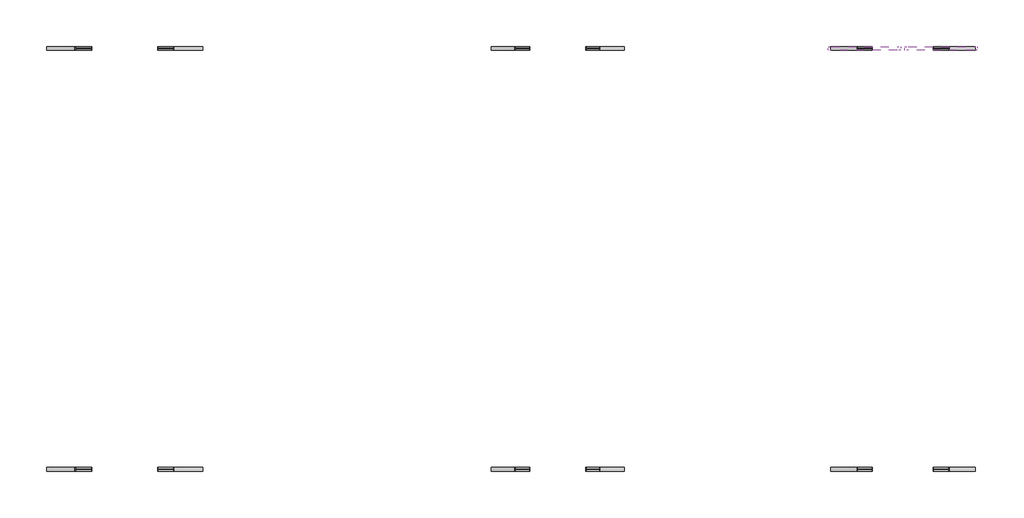
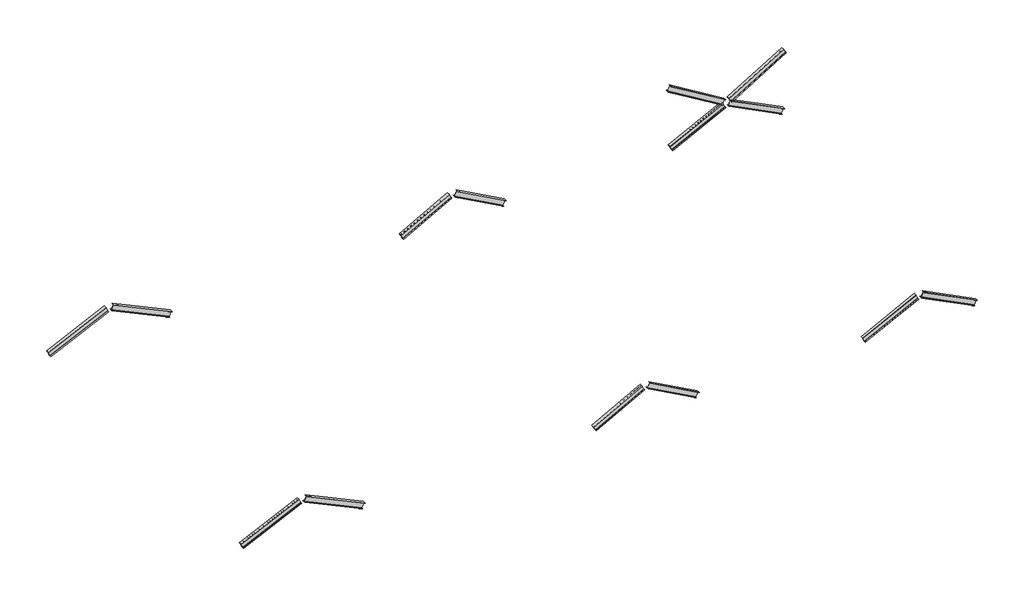
# One storey: 14 beams.
"""IFC4 building model written with IfcOpenShell, lengths in millimetres."""

import ifcopenshell
import ifcopenshell.guid

model = None  # the IFC model being written
_history = None  # IfcOwnerHistory: only IFC2X3 demands one
_inside = {}  # id of a spatial element -> (the spatial element, [elements in it])
_under = {}  # id of a project, library or spatial element -> (it, [spatial elements below it])
_declared = {}  # id of a project -> (the project, [libraries it declares])
_typed = {}  # id of a type object -> (the type object, [elements of that type])
_made_of = {}  # id of a material, layer set ... -> (it, [elements and type objects made of it])


def new_model(schema):
    """Start an empty IFC model of exactly this schema.

    Asked for "IFC4X3", IfcOpenShell would pick the latest addendum, in which some entities
    have other attributes; the version numbers below select the first issue.
    IFC2X3 requires an IfcOwnerHistory on every rooted entity: one is made here for all.
    """
    global model, _history
    if schema == "IFC4X3":
        model = ifcopenshell.file(schema_version=(4, 3, 0, 0))
    else:
        model = ifcopenshell.file(schema=schema)
    _inside.clear()
    _under.clear()
    _declared.clear()
    _typed.clear()
    _made_of.clear()
    _history = None
    if model.schema == "IFC2X3":
        org = make("IfcOrganization", Name="unknown")
        user = make(
            "IfcPersonAndOrganization",
            ThePerson=make("IfcPerson", FamilyName="unknown"),
            TheOrganization=org,
        )
        app = make(
            "IfcApplication",
            ApplicationDeveloper=org,
            Version="unknown",
            ApplicationFullName="unknown",
            ApplicationIdentifier="unknown",
        )
        _history = make(
            "IfcOwnerHistory",
            OwningUser=user,
            OwningApplication=app,
            ChangeAction="ADDED",
            CreationDate=0,
        )
    return model


def make(cls, **values):
    """One entity of the class cls with the attributes given. An attribute that is None is left unset."""
    return model.create_entity(
        cls, **{name: value for name, value in values.items() if value is not None}
    )


def rooted(cls, **values):
    """An entity with a GlobalId (a new one), such as an element, a storey or a relation."""
    return make(cls, GlobalId=ifcopenshell.guid.new(), OwnerHistory=_history, **values)


def si_unit(unit_type, name, prefix=None):
    """IfcSIUnit, for example si_unit("LENGTHUNIT", "METRE", prefix="MILLI")."""
    return make("IfcSIUnit", UnitType=unit_type, Prefix=prefix, Name=name)


def assignment(units):
    """IfcUnitAssignment: the units of a project."""
    return None if units is None else make("IfcUnitAssignment", Units=units)


def point(xyz):
    """IfcCartesianPoint."""
    return None if xyz is None else make("IfcCartesianPoint", Coordinates=xyz)


def direction(xyz):
    """IfcDirection."""
    return None if xyz is None else make("IfcDirection", DirectionRatios=xyz)


def frame(location, z_axis=None, x_axis=None):
    """IfcAxis2Placement3D, a coordinate frame: its origin and axes. An axis left out is left unset."""
    return make(
        "IfcAxis2Placement3D",
        Location=point(location),
        Axis=direction(z_axis),
        RefDirection=direction(x_axis),
    )


def frame_2d(location, x_axis=None):
    """IfcAxis2Placement2D, a coordinate frame in the plane: its origin and x axis."""
    return make(
        "IfcAxis2Placement2D", Location=point(location), RefDirection=direction(x_axis)
    )


def origin():
    """The frame at (0, 0, 0) with its axes left unset."""
    return frame((0.0, 0.0, 0.0))


def place(relative_to, where):
    """IfcLocalPlacement: puts the frame where relative to a parent placement (None: the world)."""
    return make(
        "IfcLocalPlacement", PlacementRelTo=relative_to, RelativePlacement=where
    )


def context(
    kind, dimensions, precision=None, world=None, true_north=None, identifier=None
):
    """IfcGeometricRepresentationContext, for example the 3D "Model" context."""
    return make(
        "IfcGeometricRepresentationContext",
        ContextIdentifier=identifier,
        ContextType=kind,
        CoordinateSpaceDimension=dimensions,
        Precision=precision,
        WorldCoordinateSystem=world,
        TrueNorth=true_north,
    )


def project(units=None, contexts=None):
    """IfcProject with its units and contexts."""
    return rooted(
        "IfcProject",
        Name="project",
        RepresentationContexts=contexts,
        UnitsInContext=assignment(units),
    )


def spatial(cls, under=None, at=None, **own):
    """A site, building, storey or space (cls), placed at a placement, below another one or the project."""
    s = rooted(cls, ObjectPlacement=at, **own)
    if under is not None:
        _under.setdefault(under.id(), (under, []))[1].append(s)
    return s


def polyline(points):
    """IfcPolyline through the points."""
    return make("IfcPolyline", Points=[point(p) for p in points])


def circle_curve(where, radius):
    """IfcCircle in the frame where."""
    return make("IfcCircle", Position=where, Radius=radius)


def trimmed(basis, trim1, trim2, sense, master):
    """IfcTrimmedCurve: the piece of a basis curve between two trims."""
    return make(
        "IfcTrimmedCurve",
        BasisCurve=basis,
        Trim1=trim1,
        Trim2=trim2,
        SenseAgreement=sense,
        MasterRepresentation=master,
    )


def segment(curve, same_sense, transition):
    """IfcCompositeCurveSegment."""
    return make(
        "IfcCompositeCurveSegment",
        Transition=transition,
        SameSense=same_sense,
        ParentCurve=curve,
    )


def composite_curve(segments, self_intersect=None):
    """IfcCompositeCurve: segments joined end to end."""
    return make("IfcCompositeCurve", Segments=segments, SelfIntersect=self_intersect)


def outline(outer, holes=None, kind="AREA"):
    """IfcArbitraryClosedProfileDef: a profile drawn as a closed curve; with holes, ...WithVoids."""
    if holes is None:
        return make("IfcArbitraryClosedProfileDef", ProfileType=kind, OuterCurve=outer)
    return make(
        "IfcArbitraryProfileDefWithVoids",
        ProfileType=kind,
        OuterCurve=outer,
        InnerCurves=holes,
    )


def extrude(swept, where, along, depth):
    """IfcExtrudedAreaSolid: the profile swept, set in the frame where, extruded along a direction by depth."""
    return make(
        "IfcExtrudedAreaSolid",
        SweptArea=swept,
        Position=where,
        ExtrudedDirection=direction(along),
        Depth=depth,
    )


def shape(context_of_items, identifier, shape_type, items):
    """IfcShapeRepresentation: the items that make up one representation, for example the "Body"."""
    return make(
        "IfcShapeRepresentation",
        ContextOfItems=context_of_items,
        RepresentationIdentifier=identifier,
        RepresentationType=shape_type,
        Items=items,
    )


def source(mapping_origin, context_of_items, identifier, shape_type, items):
    """IfcRepresentationMap: a shape defined once, which mapped items show again and again."""
    return make(
        "IfcRepresentationMap",
        MappingOrigin=mapping_origin,
        MappedRepresentation=shape(context_of_items, identifier, shape_type, items),
    )


def transform(
    local_origin,
    x_axis=None,
    y_axis=None,
    z_axis=None,
    scale=None,
    scale2=None,
    scale3=None,
    uniform=True,
):
    """IfcCartesianTransformationOperator3D, or its non-uniform kind. x_axis, y_axis, z_axis: its Axis1, 2, 3."""
    if uniform:
        return make(
            "IfcCartesianTransformationOperator3D",
            Axis1=direction(x_axis),
            Axis2=direction(y_axis),
            LocalOrigin=point(local_origin),
            Scale=scale,
            Axis3=direction(z_axis),
        )
    return make(
        "IfcCartesianTransformationOperator3DnonUniform",
        Axis1=direction(x_axis),
        Axis2=direction(y_axis),
        LocalOrigin=point(local_origin),
        Scale=scale,
        Axis3=direction(z_axis),
        Scale2=scale2,
        Scale3=scale3,
    )


def mapped(mapping_source, mapping_target):
    """IfcMappedItem: shows the shape of a source again, moved by a transform."""
    return make(
        "IfcMappedItem", MappingSource=mapping_source, MappingTarget=mapping_target
    )


def made_of(thing, what):
    """Note that an element or type object is made of a material, layer set ...; save() writes the relation."""
    if what is not None:
        _made_of.setdefault(what.id(), (what, []))[1].append(thing)
    return thing


def element(
    cls,
    number,
    at=None,
    inside=None,
    cuts=None,
    type_object=None,
    material=None,
    context=None,
    identifier="Body",
    shape_type=None,
    held_by="IfcProductDefinitionShape",
    body=None,
    shapes=None,
    **own,
):
    """One element of the class cls, such as IfcWall. Its Tag is "e" and its number.

    at: its placement. inside: the storey or other place that contains it. cuts: it is an
    opening in that element (IfcRelVoidsElement). A single representation is given by context,
    identifier, shape_type and body (its items); several are given by shapes. held_by: the class
    of the entity that holds the representations. save() writes the other relations.
    """
    e = rooted(cls, Tag="e%d" % number, ObjectPlacement=at, **own)
    if body is not None:
        shapes = [shape(context, identifier, shape_type, body)]
    if shapes is not None:
        e.Representation = make(held_by, Representations=shapes)
    if inside is not None:
        _inside.setdefault(inside.id(), (inside, []))[1].append(e)
    if cuts is not None:
        rooted(
            "IfcRelVoidsElement", RelatingBuildingElement=cuts, RelatedOpeningElement=e
        )
    if type_object is not None:
        _typed.setdefault(type_object.id(), (type_object, []))[1].append(e)
    return made_of(e, material)


def aggregate(whole, parts):
    """IfcRelAggregates: a whole, such as a stair, and the parts it consists of."""
    return rooted("IfcRelAggregates", RelatingObject=whole, RelatedObjects=parts)


def save(model, path):
    """Write the relations noted so far, then the file.

    IfcRelAggregates (storeys below a building ...), IfcRelContainedInSpatialStructure (elements
    in a storey), IfcRelDefinesByType, IfcRelAssociatesMaterial and IfcRelDeclares: one each for
    every whole, place, type object, material and project.
    """
    for whole, parts in _under.values():
        aggregate(whole, parts)
    for where, things in _inside.values():
        rooted(
            "IfcRelContainedInSpatialStructure",
            RelatedElements=things,
            RelatingStructure=where,
        )
    for kind, things in _typed.values():
        rooted("IfcRelDefinesByType", RelatedObjects=things, RelatingType=kind)
    for what, things in _made_of.values():
        rooted("IfcRelAssociatesMaterial", RelatedObjects=things, RelatingMaterial=what)
    for by, libraries in _declared.values():
        rooted("IfcRelDeclares", RelatingContext=by, RelatedDefinitions=libraries)
    model.write(path)


def beam_b71a2e39(model_context):
    return source(origin(), model_context, "Body", "SweptSolid", [
        extrude(outline(composite_curve([segment(polyline([(82.5, -141.5), (82.5, -151.7), (-82.5, -151.7), (-82.5, -141.5), (-11.9, -141.5)]), True, "CONTINUOUS"), segment(trimmed(circle_curve(frame_2d((-11.9, -132.6)), 8.9), [point((-11.9, -141.5))], [point((-3.0, -132.6))], True, "CARTESIAN"), True, "CONTINUOUS"), segment(polyline([(-3.0, -132.6), (-3.0, 132.6)]), True, "CONTINUOUS"), segment(trimmed(circle_curve(frame_2d((-11.9, 132.6)), 8.9), [point((-3.0, 132.6))], [point((-11.9, 141.5))], True, "CARTESIAN"), True, "CONTINUOUS"), segment(polyline([(-11.9, 141.5), (-82.5, 141.5), (-82.5, 151.7), (82.5, 151.7), (82.5, 141.5), (11.9, 141.5)]), True, "CONTINUOUS"), segment(trimmed(circle_curve(frame_2d((11.9, 132.6)), 8.9), [point((11.9, 141.5))], [point((3.0, 132.6))], True, "CARTESIAN"), True, "CONTINUOUS"), segment(polyline([(3.0, 132.6), (3.0, -132.6)]), True, "CONTINUOUS"), segment(trimmed(circle_curve(frame_2d((11.9, -132.6)), 8.9), [point((3.0, -132.6))], [point((11.9, -141.5))], True, "CARTESIAN"), True, "CONTINUOUS"), segment(polyline([(11.9, -141.5), (82.5, -141.5)]), True, "CONTINUOUS")], self_intersect=False)), frame((-1683.7594404, 0.0, 0.0), z_axis=(1.0, 0.0, 0.0), x_axis=(0.0, 1.0, 0.0)), (0.0, 0.0, 1.0), 3450.380526),
    ])


def beam_97ed9082(model_context):
    return source(origin(), model_context, "Body", "SweptSolid", [
        extrude(outline(composite_curve([segment(polyline([(82.5, -141.5), (82.5, -151.7), (-82.5, -151.7), (-82.5, -141.5), (-11.9, -141.5)]), True, "CONTINUOUS"), segment(trimmed(circle_curve(frame_2d((-11.9, -132.6)), 8.9), [point((-11.9, -141.5))], [point((-3.0, -132.6))], True, "CARTESIAN"), True, "CONTINUOUS"), segment(polyline([(-3.0, -132.6), (-3.0, 132.6)]), True, "CONTINUOUS"), segment(trimmed(circle_curve(frame_2d((-11.9, 132.6)), 8.9), [point((-3.0, 132.6))], [point((-11.9, 141.5))], True, "CARTESIAN"), True, "CONTINUOUS"), segment(polyline([(-11.9, 141.5), (-82.5, 141.5), (-82.5, 151.7), (82.5, 151.7), (82.5, 141.5), (11.9, 141.5)]), True, "CONTINUOUS"), segment(trimmed(circle_curve(frame_2d((11.9, 132.6)), 8.9), [point((11.9, 141.5))], [point((3.0, 132.6))], True, "CARTESIAN"), True, "CONTINUOUS"), segment(polyline([(3.0, 132.6), (3.0, -132.6)]), True, "CONTINUOUS"), segment(trimmed(circle_curve(frame_2d((11.9, -132.6)), 8.9), [point((3.0, -132.6))], [point((11.9, -141.5))], True, "CARTESIAN"), True, "CONTINUOUS"), segment(polyline([(11.9, -141.5), (82.5, -141.5)]), True, "CONTINUOUS")], self_intersect=False)), frame((-1443.5851857, 0.0, 0.0), z_axis=(1.0, 0.0, 0.0), x_axis=(0.0, 1.0, 0.0)), (0.0, 0.0, 1.0), 2972.6935261),
    ])


def beam_058fccc5(model_context):
    return source(origin(), model_context, "Body", "SweptSolid", [
        extrude(outline(composite_curve([segment(polyline([(82.5, -141.5), (82.5, -151.7), (-82.5, -151.7), (-82.5, -141.5), (-11.9, -141.5)]), True, "CONTINUOUS"), segment(trimmed(circle_curve(frame_2d((-11.9, -132.6)), 8.9), [point((-11.9, -141.5))], [point((-3.0, -132.6))], True, "CARTESIAN"), True, "CONTINUOUS"), segment(polyline([(-3.0, -132.6), (-3.0, 132.6)]), True, "CONTINUOUS"), segment(trimmed(circle_curve(frame_2d((-11.9, 132.6)), 8.9), [point((-3.0, 132.6))], [point((-11.9, 141.5))], True, "CARTESIAN"), True, "CONTINUOUS"), segment(polyline([(-11.9, 141.5), (-82.5, 141.5), (-82.5, 151.7), (82.5, 151.7), (82.5, 141.5), (11.9, 141.5)]), True, "CONTINUOUS"), segment(trimmed(circle_curve(frame_2d((11.9, 132.6)), 8.9), [point((11.9, 141.5))], [point((3.0, 132.6))], True, "CARTESIAN"), True, "CONTINUOUS"), segment(polyline([(3.0, 132.6), (3.0, -132.6)]), True, "CONTINUOUS"), segment(trimmed(circle_curve(frame_2d((11.9, -132.6)), 8.9), [point((3.0, -132.6))], [point((11.9, -141.5))], True, "CARTESIAN"), True, "CONTINUOUS"), segment(polyline([(11.9, -141.5), (82.5, -141.5)]), True, "CONTINUOUS")], self_intersect=False)), frame((-1563.5376228, 0.0, 0.0), z_axis=(1.0, 0.0, 0.0), x_axis=(0.0, 1.0, 0.0)), (0.0, 0.0, 1.0), 3211.1247957),
    ])


def beam_ff0b4b27(model_context):
    return source(origin(), model_context, "Body", "SweptSolid", [
        extrude(outline(composite_curve([segment(polyline([(-82.5, -141.5), (-11.9, -141.5)]), True, "CONTINUOUS"), segment(trimmed(circle_curve(frame_2d((-11.9, -132.6)), 8.9), [point((-11.9, -141.5))], [point((-3.0, -132.6))], True, "CARTESIAN"), True, "CONTINUOUS"), segment(polyline([(-3.0, -132.6), (-3.0, 132.6)]), True, "CONTINUOUS"), segment(trimmed(circle_curve(frame_2d((-11.9, 132.6)), 8.9), [point((-3.0, 132.6))], [point((-11.9, 141.5))], True, "CARTESIAN"), True, "CONTINUOUS"), segment(polyline([(-11.9, 141.5), (-82.5, 141.5), (-82.5, 151.7), (82.5, 151.7), (82.5, 141.5), (11.9, 141.5)]), True, "CONTINUOUS"), segment(trimmed(circle_curve(frame_2d((11.9, 132.6)), 8.9), [point((11.9, 141.5))], [point((3.0, 132.6))], True, "CARTESIAN"), True, "CONTINUOUS"), segment(polyline([(3.0, 132.6), (3.0, -132.6)]), True, "CONTINUOUS"), segment(trimmed(circle_curve(frame_2d((11.9, -132.6)), 8.9), [point((3.0, -132.6))], [point((11.9, -141.5))], True, "CARTESIAN"), True, "CONTINUOUS"), segment(polyline([(11.9, -141.5), (82.5, -141.5), (82.5, -151.7), (-82.5, -151.7), (-82.5, -141.5)]), True, "CONTINUOUS")], self_intersect=False)), frame((-1737.9303669, 0.0, 0.0), z_axis=(1.0, 0.0, 0.0), x_axis=(0.0, 1.0, 0.0)), (0.0, 0.0, 1.0), 3445.4570815),
    ])


model = new_model("IFC4")

# Units and contexts
model_context = context("Model", 3, world=origin())
ifc_project = project(units=[si_unit("LENGTHUNIT", "METRE", prefix="MILLI")], contexts=[model_context])

# Site, building, storey
site = spatial("IfcSite", under=ifc_project)
building = spatial("IfcBuilding", under=site)
storey = spatial("IfcBuildingStorey", under=building, Name="G.L", Elevation=299.9720055)

# Beams
placement = place(None, origin())
beam_shape = beam_b71a2e39(model_context)
element("IfcBeam", 1, ObjectType="Old_Steel Beam_H-KSD3502 : H_SB_ASB_H-200×200x8x12", at=placement, inside=storey, context=model_context, shape_type="MappedRepresentation", body=[
    mapped(beam_shape, transform((1750.0, 20999.5208589, 1507.9720055), x_axis=(0.9051232306684414, 0.0, 0.4251493117768432), y_axis=(0.0, 1.0, 0.0), z_axis=(-0.4251493117768432, 0.0, 0.9051232306684414))),
])
element("IfcBeam", 2, ObjectType="Old_Steel Beam_H-KSD3502 : H_SB_ASB_H-200×200x8x12", at=placement, inside=storey, context=model_context, shape_type="MappedRepresentation", body=[
    mapped(beam_shape, transform((5250.0, 20999.5208589, 1507.9720055), x_axis=(-0.9051232306684284, 0.0, 0.4251493117768708), y_axis=(0.0, -1.0, 0.0), z_axis=(0.4251493117768708, 0.0, 0.9051232306684284))),
])
element("IfcBeam", 3, ObjectType="Old_Steel Beam_H-KSD3502 : H_SB_ASB_H-200×200x8x12", at=placement, inside=storey, context=model_context, shape_type="MappedRepresentation", body=[
    mapped(beam_shape, transform((1750.0, 38999.5208589, 1507.9720055), x_axis=(0.9051232306684415, 0.0, 0.4251493117768429), y_axis=(0.0, 1.0, 0.0), z_axis=(-0.4251493117768429, 0.0, 0.9051232306684415))),
])
element("IfcBeam", 4, ObjectType="Old_Steel Beam_H-KSD3502 : H_SB_ASB_H-200×200x8x12", at=placement, inside=storey, context=model_context, shape_type="MappedRepresentation", body=[
    mapped(beam_shape, transform((5250.0, 38999.5208589, 1507.9720055), x_axis=(-0.9051232306684285, 0.0, 0.4251493117768706), y_axis=(0.0, -1.0, 0.0), z_axis=(0.4251493117768706, 0.0, 0.9051232306684285))),
])
beam_2_shape = beam_97ed9082(model_context)
element("IfcBeam", 5, ObjectType="Old_Steel Beam_H-KSD3502 : H_SB_ASB_H-200×200x8x12", at=placement, inside=storey, context=model_context, shape_type="MappedRepresentation", body=[
    mapped(beam_2_shape, transform((20500.0, 20999.5208589, 1507.9720055), x_axis=(0.8769554889666458, 0.0, 0.4805716079537693), y_axis=(0.0, 1.0, 0.0), z_axis=(-0.4805716079537693, 0.0, 0.8769554889666458))),
])
element("IfcBeam", 6, ObjectType="Old_Steel Beam_H-KSD3502 : H_SB_ASB_H-200×200x8x12", at=placement, inside=storey, context=model_context, shape_type="MappedRepresentation", body=[
    mapped(beam_2_shape, transform((23500.0, 20999.5208589, 1507.9720055), x_axis=(-0.8769554889666746, 0.0, 0.4805716079537164), y_axis=(0.0, -1.0, 0.0), z_axis=(0.4805716079537164, 0.0, 0.8769554889666746))),
])
element("IfcBeam", 7, ObjectType="Old_Steel Beam_H-KSD3502 : H_SB_ASB_H-200×200x8x12", at=placement, inside=storey, context=model_context, shape_type="MappedRepresentation", body=[
    mapped(beam_2_shape, transform((20500.0, 38999.5208589, 1507.9720055), x_axis=(0.8769554889666475, 0.0, 0.4805716079537661), y_axis=(0.0, 1.0, 0.0), z_axis=(-0.4805716079537661, 0.0, 0.8769554889666475))),
])
element("IfcBeam", 8, ObjectType="Old_Steel Beam_H-KSD3502 : H_SB_ASB_H-200×200x8x12", at=placement, inside=storey, context=model_context, shape_type="MappedRepresentation", body=[
    mapped(beam_2_shape, transform((23500.0, 38999.5208589, 1507.9720055), x_axis=(-0.8769554889666732, 0.0, 0.4805716079537191), y_axis=(0.0, -1.0, 0.0), z_axis=(0.4805716079537191, 0.0, 0.8769554889666732))),
])
beam_3_shape = beam_058fccc5(model_context)
element("IfcBeam", 9, ObjectType="Old_Steel Beam_H-KSD3502 : H_SB_ASB_H-200×200x8x12", at=placement, inside=storey, context=model_context, shape_type="MappedRepresentation", body=[
    mapped(beam_3_shape, transform((38375.0, 20999.5208589, 1507.9720055), x_axis=(-0.8923307733807315, 0.0, 0.4513820896732006), y_axis=(0.0, -1.0, 0.0), z_axis=(0.4513820896732006, 0.0, 0.8923307733807315))),
])
element("IfcBeam", 10, ObjectType="Old_Steel Beam_H-KSD3502 : H_SB_ASB_H-200×200x8x12", at=placement, inside=storey, context=model_context, shape_type="MappedRepresentation", body=[
    mapped(beam_3_shape, transform((35125.0, 20999.5208589, 1507.9720055), x_axis=(0.8923307733807281, 0.0, 0.45138208967320764), y_axis=(0.0, 1.0, 0.0), z_axis=(-0.45138208967320764, 0.0, 0.8923307733807281))),
])
element("IfcBeam", 11, ObjectType="Old_Steel Beam_H-KSD3502 : H_SB_ASB_H-200×200x8x12", at=placement, inside=storey, context=model_context, shape_type="MappedRepresentation", body=[
    mapped(beam_3_shape, transform((38375.0, 38999.5208589, 1507.9720055), x_axis=(-0.8923307733807311, 0.0, 0.45138208967320154), y_axis=(0.0, -1.0, 0.0), z_axis=(0.45138208967320154, 0.0, 0.8923307733807311))),
])
element("IfcBeam", 12, ObjectType="Old_Steel Beam_H-KSD3502 : H_SB_ASB_H-200×200x8x12", at=placement, inside=storey, context=model_context, shape_type="MappedRepresentation", body=[
    mapped(beam_3_shape, transform((35125.0, 38999.5208589, 1507.9720055), x_axis=(0.8923307733807282, 0.0, 0.4513820896732074), y_axis=(0.0, 1.0, 0.0), z_axis=(-0.4513820896732074, 0.0, 0.8923307733807282))),
])
beam_4_shape = beam_ff0b4b27(model_context)
element("IfcBeam", 13, ObjectType="Old_Steel Beam_H-KSD3502 : H_SB_ASB_H-200×200x8x12", at=placement, inside=storey, context=model_context, shape_type="MappedRepresentation", body=[
    mapped(beam_4_shape, transform((38375.0, 38999.5208589, 3314.1220055), x_axis=(-0.855360757222787, 0.0, -0.518032793366656), y_axis=(0.0, -1.0, 0.0), z_axis=(-0.518032793366656, 0.0, 0.855360757222787))),
])
element("IfcBeam", 14, ObjectType="Old_Steel Beam_H-KSD3502 : H_SB_ASB_H-200×200x8x12", at=placement, inside=storey, context=model_context, shape_type="MappedRepresentation", body=[
    mapped(beam_4_shape, transform((35125.0, 38999.5208589, 3314.1220055), x_axis=(0.8553607572227874, 0.0, -0.5180327933666553), y_axis=(0.0, 1.0, 0.0), z_axis=(0.5180327933666553, 0.0, 0.8553607572227874))),
])

save(model, "model.ifc")

# Revit data of these elements
# Type "Old_Steel Beam_H-KSD3502 : H_SB_ASB_H-200×200x8x12"
#   Width = 20.0 cm
#   Web Thickness = 0.8 cm
#   Web Fillet = 1.3 cm
#   Warping Constant = 141376.0 cm⁶
#   Torsional Moment of Inertia = 26.2485 cm⁴
#   Torsional Modulus = 1.0 cm³
#   Section Area = 63.53 cm²
#   Plastic Modulus weak axis = 244.0 cm³
#   Plastic Modulus strong axis = 525.0 cm³
#   Perimeter = 1.16 m²/m
#   Nominal Weight = 49.90 kgf/m
#   Moment of Inertia weak axis = 1600.00 cm⁴
#   Moment of Inertia strong axis = 4720.00 cm⁴
#   Height = 20.0 cm
#   Flange Thickness = 1.2 cm
#   Elastic Modulus weak axis = 160.0 cm³
#   Elastic Modulus strong axis = 472.0 cm³
#   Centroid Vertical = 10.0 cm
#   Centroid Horizontal = 10.0 cm
#   Length [instance default] = 1.5240 m
#   Structural Material [instance default] = Steel, 45-345
#   Assembly Code = ""
# Elements 1, 2, 5, 6, 9, 10 (IfcBeam, "Old_Steel Beam_H-KSD3502 : H_SB_ASB_H-200×200x8x12")
#   Mark = "VB1"
#   LINE SCHEDULE = "A"
#   Structural Material = none
#   Phase Created = New Construction
# Elements 3, 4, 7, 8, 11, 12, 13, 14 (IfcBeam, "Old_Steel Beam_H-KSD3502 : H_SB_ASB_H-200×200x8x12")
#   Mark = "VB1"
#   Structural Material = none
#   Phase Created = New Construction
# Materials
#   "Steel, 45-345": class "Metal", colour RGB 189 187 185, transparency 0, Description = "Steel 345 MPa", Cost = 0
